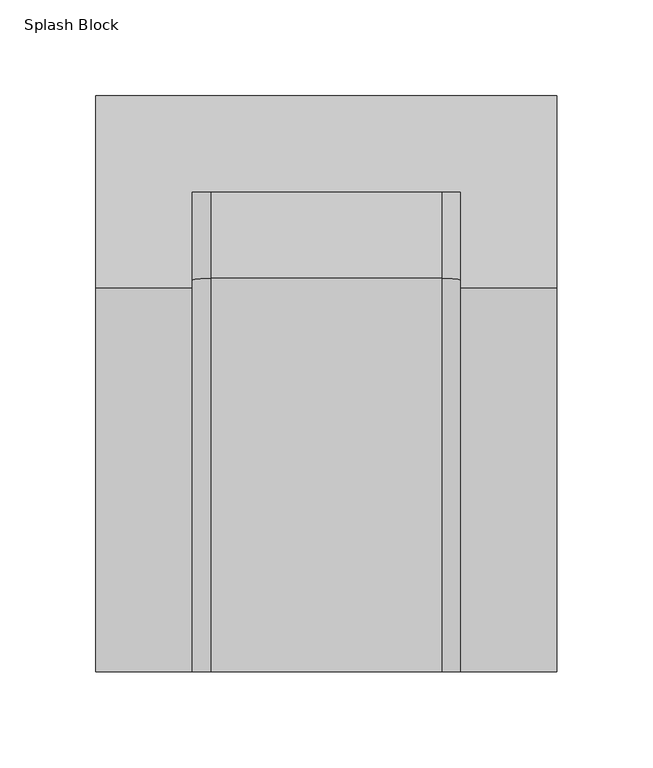
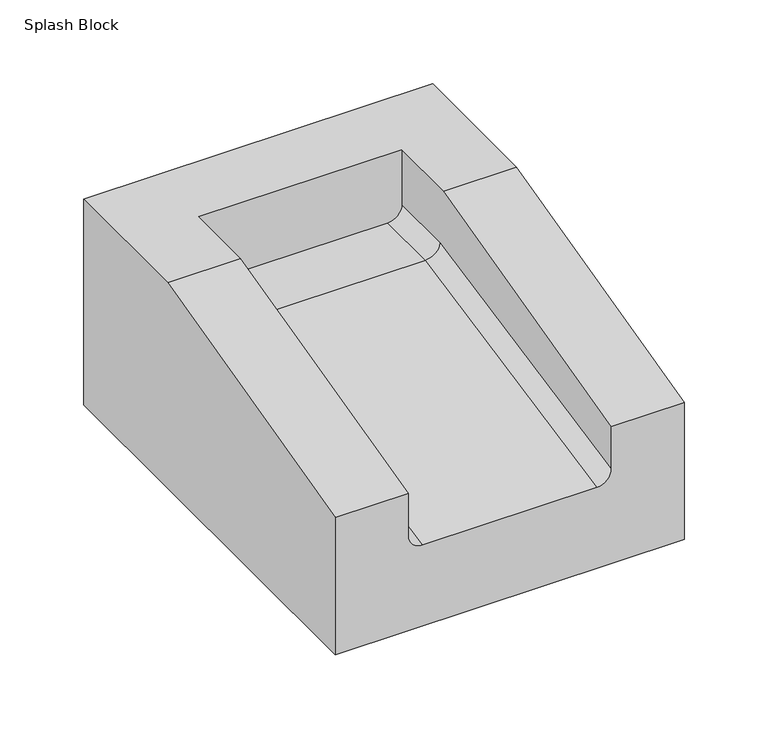
"""IFC4 building model written with IfcOpenShell, lengths in millimetres: proxy geometry, Splash Block : H_GM_AR_B07_Splash Block_240x300."""

from ifc_helpers import new_model, si_unit, frame, origin, place, context, project, spatial, polyline, circle_curve, ellipse_curve, source, transform, mapped, element, save
from ifc_brep_helpers import plane_surface, revolved_surface, advanced_brep


def splash_block_9e3ddbbe(model_context):
    return source(origin(), model_context, "Body", "AdvancedBrep", [
        advanced_brep(
        [(120.0, 0.0, 150.0), (120.0, -100.0, 150.0), (120.0, -300.0, 100.0), (120.0, -300.0, 0.0), (120.0, 0.0, 0.0), (-120.0, 0.0, 150.0), (-120.0, 0.0, 0.0), (-120.0, -300.0, 0.0), (-120.0, -300.0, 100.0), (-120.0, -100.0, 150.0), (-70.0, -100.0, 150.0), (-70.0, -50.0, 150.0), (70.0, -50.0, 150.0), (70.0, -100.0, 150.0), (70.0, -300.0, 100.0), (-70.0, -300.0, 100.0), (70.0, -300.0, 69.2078439), (60.0, -300.0, 59.0098049), (-60.0, -300.0, 59.0098049), (-70.0, -300.0, 69.2078439), (60.0, -50.0, 100.0), (70.0, -50.0, 110.0), (-70.0, -50.0, 110.0), (-60.0, -50.0, 100.0), (70.0, -96.0392195, 110.0), (-70.0, -96.0392195, 110.0), (60.0, -95.0490243, 100.0), (-60.0, -95.0490243, 100.0)],
        [
            (0, 1),
            (1, 2),
            (2, 3),
            (3, 4),
            (4, 0),
            (5, 6),
            (6, 7),
            (7, 8),
            (8, 9),
            (9, 5),
            (0, 5),
            (9, 10),
            (10, 11),
            (11, 12),
            (12, 13),
            (13, 1),
            (13, 14),
            (14, 2),
            (8, 15),
            (15, 10),
            (14, 16),
            (16, 17, ellipse_curve(frame((60.0, -300.0, 69.2078439), z_axis=(0.0, 1.0, 0.0), x_axis=(0.0, 0.0, -1.0)), 10.198039, 10.0)),
            (17, 18),
            (18, 19, ellipse_curve(frame((-60.0, -300.0, 69.2078439), z_axis=(0.0, 1.0, 0.0), x_axis=(0.0, 0.0, -1.0)), 10.198039, 10.0)),
            (19, 15),
            (7, 3),
            (6, 4),
            (20, 21, circle_curve(frame((60.0, -50.0, 110.0), z_axis=(0.0, -1.0, 0.0), x_axis=(0.0, 0.0, 1.0)), 10.0)),
            (21, 12),
            (11, 22),
            (22, 23, circle_curve(frame((-60.0, -50.0, 110.0), z_axis=(0.0, -1.0, 0.0), x_axis=(0.0, 0.0, 1.0)), 10.0)),
            (23, 20),
            (21, 24),
            (24, 16),
            (19, 25),
            (25, 22),
            (26, 27),
            (27, 18),
            (17, 26),
            (23, 27),
            (26, 20),
            (24, 26, ellipse_curve(frame((60.0, -96.0392195, 110.0), z_axis=(0.0, 0.9951333266680704, 0.09853761796664144), x_axis=(0.0, 0.09853761796664429, -0.99513332666807)), 10.0489047, 10.0)),
            (27, 25, ellipse_curve(frame((-60.0, -96.0392195, 110.0), z_axis=(0.0, 0.9951333266680704, 0.09853761796664144), x_axis=(0.0, 0.09853761796664429, -0.99513332666807)), 10.0489047, 10.0)),
        ],
        [
            plane_surface(frame((120.0, 0.0, 150.0), z_axis=(1.0, 0.0, 0.0), x_axis=(0.0, -1.0, 0.0))),
            plane_surface(frame((-120.0, 0.0, 150.0), z_axis=(-1.0, 0.0, 0.0), x_axis=(0.0, 1.0, 0.0))),
            plane_surface(frame((120.0, 0.0, 150.0), z_axis=(0.0, 0.0, 1.0), x_axis=(-1.0, 0.0, 0.0))),
            plane_surface(frame((120.0, -100.0, 150.0), z_axis=(0.0, -0.2425356250363336, 0.9701425001453318), x_axis=(-1.0, 0.0, 0.0))),
            plane_surface(frame((120.0, -300.0, 100.0), z_axis=(0.0, -1.0, 0.0), x_axis=(-1.0, 0.0, 0.0))),
            plane_surface(frame((120.0, -300.0, 0.0), z_axis=(0.0, 0.0, -1.0), x_axis=(-1.0, 0.0, 0.0))),
            plane_surface(frame((120.0, 0.0, 0.0), z_axis=(0.0, 1.0, 0.0), x_axis=(-1.0, 0.0, 0.0))),
            plane_surface(frame((0.0, -50.0, 100.0), z_axis=(0.0, -1.0, 0.0), x_axis=(1.0, 0.0, 0.0))),
            plane_surface(frame((70.0, -351.9611614, 58.8156116), z_axis=(-1.0, 0.0, 0.0), x_axis=(0.0, 0.9805806756909198, 0.19611613513818588))),
            plane_surface(frame((-70.0, -359.8058068, 98.0388386), z_axis=(1.0, 0.0, 0.0), x_axis=(0.0, 0.9805806756909198, 0.19611613513818585))),
            plane_surface(frame((-60.0, -350.0, 49.0098049), z_axis=(0.0, -0.1961161351381859, 0.9805806756909199), x_axis=(0.0, 0.9805806756909199, 0.1961161351381859))),
            plane_surface(frame((-60.0, -95.0490243, 100.0), z_axis=(0.0, 0.0, 1.0), x_axis=(0.0, 1.0, 0.0))),
            revolved_surface(polyline([(60.0, -303.9223226936896, 78.62141836844775), (60.0, -97.02941463562763, 119.99999998006055)]), (60.0, -351.9611614, 58.8156116), (0.0, -0.9805806756909199, -0.1961161351381859)),
            revolved_surface(polyline([(-60.0, -303.9223226936896, 78.62141836844775), (-60.0, -97.02941463562763, 119.99999998006055)]), (-60.0, -351.9611614, 58.8156116), (0.0, -0.9805806756909199, -0.1961161351381859)),
            revolved_surface(polyline([(60.0, -97.02941463231181, 120.0), (60.0, -50.0, 120.0)]), (60.0, -95.0490243, 110.0), (0.0, -1.0, 0.0)),
            revolved_surface(polyline([(-60.0, -97.02941463231181, 120.0), (-60.0, -50.0, 120.0)]), (-60.0, -95.0490243, 110.0), (0.0, -1.0, 0.0)),
        ],
        [
            (0, [[1, 2, 3, 4, 5]]),
            (1, [[6, 7, 8, 9, 10]]),
            (2, [[-1, 11, -10, 12, 13, 14, 15, 16]]),
            (3, [[-2, -16, 17, 18]]),
            (3, [[-9, 19, 20, -12]]),
            (4, [[-3, -18, 21, 22, 23, 24, 25, -19, -8, 26]]),
            (5, [[-4, -26, -7, 27]]),
            (6, [[-5, -27, -6, -11]]),
            (7, [[28, 29, -14, 30, 31, 32]]),
            (8, [[-29, 33, 34, -21, -17, -15]]),
            (9, [[-30, -13, -20, -25, 35, 36]]),
            (10, [[37, 38, -23, 39]]),
            (11, [[-32, 40, -37, 41]]),
            (12, [[42, -39, -22, -34]]),
            (13, [[43, -35, -24, -38]]),
            (14, [[-28, -41, -42, -33]]),
            (15, [[-31, -36, -43, -40]]),
        ],
    ),
    ])


if __name__ == "__main__":
    model = new_model("IFC4")
    model_context = context("Model", 3, world=origin())
    ifc_project = project(units=[si_unit("LENGTHUNIT", "METRE", prefix="MILLI")], contexts=[model_context])
    site = spatial("IfcSite", under=ifc_project)
    building = spatial("IfcBuilding", under=site)
    placement = place(None, origin())
    splash_block_shape = splash_block_9e3ddbbe(model_context)
    element("IfcBuildingElementProxy", 1, Name="Splash Block : H_GM_AR_B07_Splash Block_240x300", ObjectType="Splash Block : H_GM_AR_B07_Splash Block_240x300", at=placement, inside=building, context=model_context, shape_type="MappedRepresentation", body=[
        mapped(splash_block_shape, transform((0.0, 0.0, 0.0), x_axis=(1.0, 0.0, 0.0), y_axis=(0.0, 1.0, 0.0), z_axis=(0.0, 0.0, 1.0))),
    ])
    save(model, "model.ifc")

# Revit data of these elements
# Type "Splash Block : H_GM_AR_B07_Splash Block_240x300"
#   Width [instance default] = 240 mm
#   Length [instance default] = 350 mm
#   Material [instance default] = none
#   Default Elevation = 0
# Element 1 (IfcBuildingElementProxy, "Splash Block : H_GM_AR_B07_Splash Block_240x300")
#   Length = 300 mm
